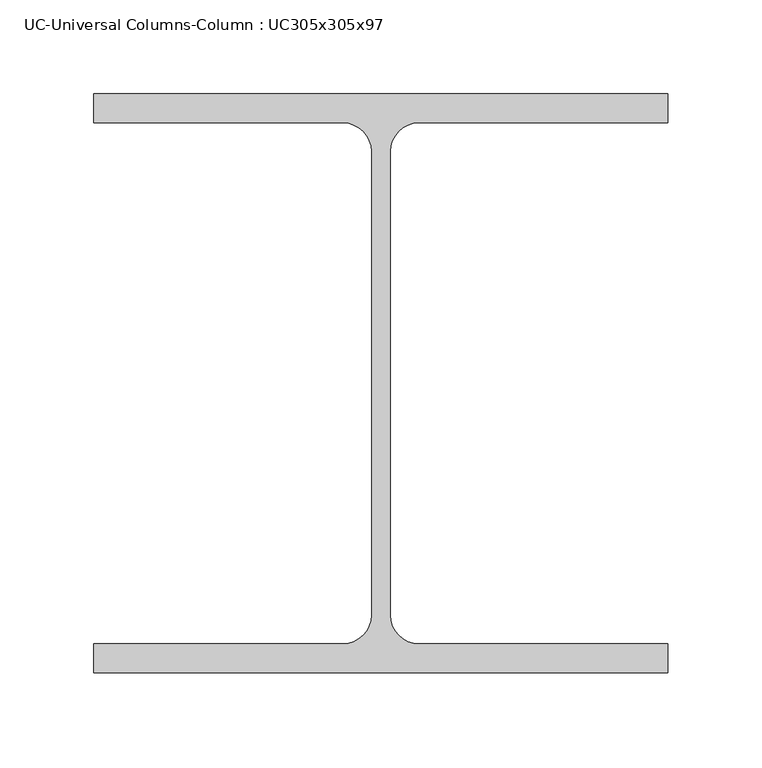
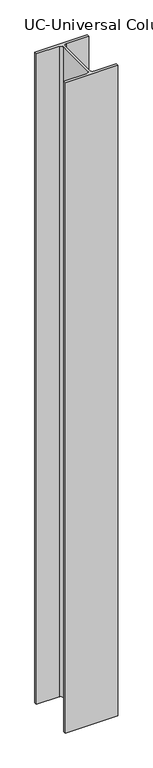
"""IFC4 building model written with IfcOpenShell, lengths in millimetres: column geometry, UC-Universal Columns-Column : UC305x305x97."""

from ifc_helpers import new_model, si_unit, point, frame_2d, origin, origin_with_axes, place, context, project, spatial, polyline, circle_curve, trimmed, segment, composite_curve, outline, extrude, source, transform, mapped, element, save


def uc_universal_columns_column_uc305x305x97_9aa56e74(model_context):
    return source(origin(), model_context, "Body", "SweptSolid", [
        extrude(outline(composite_curve([segment(polyline([(152.65, 153.95), (152.65, 138.55), (20.15, 138.55)]), True, "CONTINUOUS"), segment(trimmed(circle_curve(frame_2d((20.15, 123.35)), 15.2), [point((20.15, 138.55))], [point((4.95, 123.35))], True, "CARTESIAN"), True, "CONTINUOUS"), segment(polyline([(4.95, 123.35), (4.95, -123.35)]), True, "CONTINUOUS"), segment(trimmed(circle_curve(frame_2d((20.15, -123.35)), 15.2), [point((4.95, -123.35))], [point((20.15, -138.55))], True, "CARTESIAN"), True, "CONTINUOUS"), segment(polyline([(20.15, -138.55), (152.65, -138.55), (152.65, -153.95), (-152.65, -153.95), (-152.65, -138.55), (-20.15, -138.55)]), True, "CONTINUOUS"), segment(trimmed(circle_curve(frame_2d((-20.15, -123.35)), 15.2), [point((-20.15, -138.55))], [point((-4.95, -123.35))], True, "CARTESIAN"), True, "CONTINUOUS"), segment(polyline([(-4.95, -123.35), (-4.95, 123.35)]), True, "CONTINUOUS"), segment(trimmed(circle_curve(frame_2d((-20.15, 123.35)), 15.2), [point((-4.95, 123.35))], [point((-20.15, 138.55))], True, "CARTESIAN"), True, "CONTINUOUS"), segment(polyline([(-20.15, 138.55), (-152.65, 138.55), (-152.65, 153.95), (152.65, 153.95)]), True, "CONTINUOUS")], self_intersect=False)), origin_with_axes(), (0.0, 0.0, 1.0), 4000.0),
    ])


if __name__ == "__main__":
    model = new_model("IFC4")
    model_context = context("Model", 3, world=origin())
    ifc_project = project(units=[si_unit("LENGTHUNIT", "METRE", prefix="MILLI")], contexts=[model_context])
    site = spatial("IfcSite", under=ifc_project)
    building = spatial("IfcBuilding", under=site)
    placement = place(None, origin())
    uc_universal_columns_column_uc305x305x97_shape = uc_universal_columns_column_uc305x305x97_9aa56e74(model_context)
    element("IfcColumn", 1, ObjectType="UC-Universal Columns-Column : UC305x305x97", at=placement, inside=building, context=model_context, shape_type="MappedRepresentation", body=[
        mapped(uc_universal_columns_column_uc305x305x97_shape, transform((0.0, 0.0, 0.0), x_axis=(1.0, 0.0, 0.0), y_axis=(0.0, 1.0, 0.0), z_axis=(0.0, 0.0, 1.0))),
    ])
    save(model, "model.ifc")

# Revit data of these elements
# Type "UC-Universal Columns-Column : UC305x305x97"
#   Section Name Key = "UC305x305x97"
#   Width = 30.53 cm
#   Web Thickness = 0.99 cm
#   Web Fillet = 1.52 cm
#   Warping Constant = 1560000.0 cm⁶
#   Torsional Moment of Inertia = 91.20 cm⁴
#   Section Area = 123.0 cm²
#   Plastic Modulus weak axis = 726.0 cm³
#   Plastic Modulus strong axis = 1592.0 cm³
#   Nominal Weight = 96.8996 kgf/m
#   Moment of Inertia weak axis = 7308.00 cm⁴
#   Moment of Inertia strong axis = 22249.00 cm⁴
#   Height = 30.79 cm
#   Flange Thickness = 1.54 cm
#   Elastic Modulus weak axis = 479.0 cm³
#   Elastic Modulus strong axis = 1445.0 cm³
#   Centroid Vertical = 15.395 cm
#   Centroid Horizontal = 15.265 cm
#   Bolt Spacing = 14.0 cm
#   Structural Material [instance default] = Metal - Steel 43-275
#   Type Comments = ""
#   Assembly Code = ""
# Element 1 (IfcColumn, "UC-Universal Columns-Column : UC305x305x97")
#   Materials on its faces: "Metal - Steel 43-275"
# Materials
#   "Metal - Steel 43-275": class "Metal", colour RGB 247 247 247, transparency 0, Cost = 0
